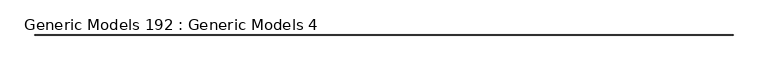
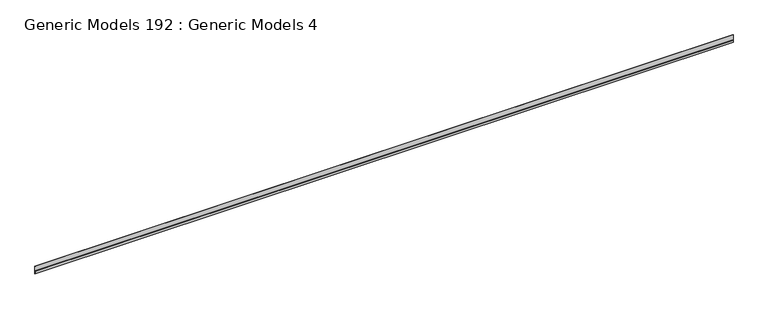
"""IFC4 building model written with IfcOpenShell, lengths in millimetres: proxy geometry, Generic Models 192 : Generic Models 4."""

import ifcopenshell
import ifcopenshell.guid

model = None  # the IFC model being written
_history = None  # IfcOwnerHistory: only IFC2X3 demands one
_inside = {}  # id of a spatial element -> (the spatial element, [elements in it])
_under = {}  # id of a project, library or spatial element -> (it, [spatial elements below it])
_declared = {}  # id of a project -> (the project, [libraries it declares])
_typed = {}  # id of a type object -> (the type object, [elements of that type])
_made_of = {}  # id of a material, layer set ... -> (it, [elements and type objects made of it])


def new_model(schema):
    """Start an empty IFC model of exactly this schema.

    Asked for "IFC4X3", IfcOpenShell would pick the latest addendum, in which some entities
    have other attributes; the version numbers below select the first issue.
    IFC2X3 requires an IfcOwnerHistory on every rooted entity: one is made here for all.
    """
    global model, _history
    if schema == "IFC4X3":
        model = ifcopenshell.file(schema_version=(4, 3, 0, 0))
    else:
        model = ifcopenshell.file(schema=schema)
    _inside.clear()
    _under.clear()
    _declared.clear()
    _typed.clear()
    _made_of.clear()
    _history = None
    if model.schema == "IFC2X3":
        org = make("IfcOrganization", Name="unknown")
        user = make(
            "IfcPersonAndOrganization",
            ThePerson=make("IfcPerson", FamilyName="unknown"),
            TheOrganization=org,
        )
        app = make(
            "IfcApplication",
            ApplicationDeveloper=org,
            Version="unknown",
            ApplicationFullName="unknown",
            ApplicationIdentifier="unknown",
        )
        _history = make(
            "IfcOwnerHistory",
            OwningUser=user,
            OwningApplication=app,
            ChangeAction="ADDED",
            CreationDate=0,
        )
    return model


def make(cls, **values):
    """One entity of the class cls with the attributes given. An attribute that is None is left unset."""
    return model.create_entity(
        cls, **{name: value for name, value in values.items() if value is not None}
    )


def rooted(cls, **values):
    """An entity with a GlobalId (a new one), such as an element, a storey or a relation."""
    return make(cls, GlobalId=ifcopenshell.guid.new(), OwnerHistory=_history, **values)


def si_unit(unit_type, name, prefix=None):
    """IfcSIUnit, for example si_unit("LENGTHUNIT", "METRE", prefix="MILLI")."""
    return make("IfcSIUnit", UnitType=unit_type, Prefix=prefix, Name=name)


def assignment(units):
    """IfcUnitAssignment: the units of a project."""
    return None if units is None else make("IfcUnitAssignment", Units=units)


def point(xyz):
    """IfcCartesianPoint."""
    return None if xyz is None else make("IfcCartesianPoint", Coordinates=xyz)


def direction(xyz):
    """IfcDirection."""
    return None if xyz is None else make("IfcDirection", DirectionRatios=xyz)


def frame(location, z_axis=None, x_axis=None):
    """IfcAxis2Placement3D, a coordinate frame: its origin and axes. An axis left out is left unset."""
    return make(
        "IfcAxis2Placement3D",
        Location=point(location),
        Axis=direction(z_axis),
        RefDirection=direction(x_axis),
    )


def origin():
    """The frame at (0, 0, 0) with its axes left unset."""
    return frame((0.0, 0.0, 0.0))


def place(relative_to, where):
    """IfcLocalPlacement: puts the frame where relative to a parent placement (None: the world)."""
    return make(
        "IfcLocalPlacement", PlacementRelTo=relative_to, RelativePlacement=where
    )


def context(
    kind, dimensions, precision=None, world=None, true_north=None, identifier=None
):
    """IfcGeometricRepresentationContext, for example the 3D "Model" context."""
    return make(
        "IfcGeometricRepresentationContext",
        ContextIdentifier=identifier,
        ContextType=kind,
        CoordinateSpaceDimension=dimensions,
        Precision=precision,
        WorldCoordinateSystem=world,
        TrueNorth=true_north,
    )


def project(units=None, contexts=None):
    """IfcProject with its units and contexts."""
    return rooted(
        "IfcProject",
        Name="project",
        RepresentationContexts=contexts,
        UnitsInContext=assignment(units),
    )


def spatial(cls, under=None, at=None, **own):
    """A site, building, storey or space (cls), placed at a placement, below another one or the project."""
    s = rooted(cls, ObjectPlacement=at, **own)
    if under is not None:
        _under.setdefault(under.id(), (under, []))[1].append(s)
    return s


def polyline(points):
    """IfcPolyline through the points."""
    return make("IfcPolyline", Points=[point(p) for p in points])


def outline(outer, holes=None, kind="AREA"):
    """IfcArbitraryClosedProfileDef: a profile drawn as a closed curve; with holes, ...WithVoids."""
    if holes is None:
        return make("IfcArbitraryClosedProfileDef", ProfileType=kind, OuterCurve=outer)
    return make(
        "IfcArbitraryProfileDefWithVoids",
        ProfileType=kind,
        OuterCurve=outer,
        InnerCurves=holes,
    )


def extrude(swept, where, along, depth):
    """IfcExtrudedAreaSolid: the profile swept, set in the frame where, extruded along a direction by depth."""
    return make(
        "IfcExtrudedAreaSolid",
        SweptArea=swept,
        Position=where,
        ExtrudedDirection=direction(along),
        Depth=depth,
    )


def shape(context_of_items, identifier, shape_type, items):
    """IfcShapeRepresentation: the items that make up one representation, for example the "Body"."""
    return make(
        "IfcShapeRepresentation",
        ContextOfItems=context_of_items,
        RepresentationIdentifier=identifier,
        RepresentationType=shape_type,
        Items=items,
    )


def source(mapping_origin, context_of_items, identifier, shape_type, items):
    """IfcRepresentationMap: a shape defined once, which mapped items show again and again."""
    return make(
        "IfcRepresentationMap",
        MappingOrigin=mapping_origin,
        MappedRepresentation=shape(context_of_items, identifier, shape_type, items),
    )


def transform(
    local_origin,
    x_axis=None,
    y_axis=None,
    z_axis=None,
    scale=None,
    scale2=None,
    scale3=None,
    uniform=True,
):
    """IfcCartesianTransformationOperator3D, or its non-uniform kind. x_axis, y_axis, z_axis: its Axis1, 2, 3."""
    if uniform:
        return make(
            "IfcCartesianTransformationOperator3D",
            Axis1=direction(x_axis),
            Axis2=direction(y_axis),
            LocalOrigin=point(local_origin),
            Scale=scale,
            Axis3=direction(z_axis),
        )
    return make(
        "IfcCartesianTransformationOperator3DnonUniform",
        Axis1=direction(x_axis),
        Axis2=direction(y_axis),
        LocalOrigin=point(local_origin),
        Scale=scale,
        Axis3=direction(z_axis),
        Scale2=scale2,
        Scale3=scale3,
    )


def mapped(mapping_source, mapping_target):
    """IfcMappedItem: shows the shape of a source again, moved by a transform."""
    return make(
        "IfcMappedItem", MappingSource=mapping_source, MappingTarget=mapping_target
    )


def made_of(thing, what):
    """Note that an element or type object is made of a material, layer set ...; save() writes the relation."""
    if what is not None:
        _made_of.setdefault(what.id(), (what, []))[1].append(thing)
    return thing


def element(
    cls,
    number,
    at=None,
    inside=None,
    cuts=None,
    type_object=None,
    material=None,
    context=None,
    identifier="Body",
    shape_type=None,
    held_by="IfcProductDefinitionShape",
    body=None,
    shapes=None,
    **own,
):
    """One element of the class cls, such as IfcWall. Its Tag is "e" and its number.

    at: its placement. inside: the storey or other place that contains it. cuts: it is an
    opening in that element (IfcRelVoidsElement). A single representation is given by context,
    identifier, shape_type and body (its items); several are given by shapes. held_by: the class
    of the entity that holds the representations. save() writes the other relations.
    """
    e = rooted(cls, Tag="e%d" % number, ObjectPlacement=at, **own)
    if body is not None:
        shapes = [shape(context, identifier, shape_type, body)]
    if shapes is not None:
        e.Representation = make(held_by, Representations=shapes)
    if inside is not None:
        _inside.setdefault(inside.id(), (inside, []))[1].append(e)
    if cuts is not None:
        rooted(
            "IfcRelVoidsElement", RelatingBuildingElement=cuts, RelatedOpeningElement=e
        )
    if type_object is not None:
        _typed.setdefault(type_object.id(), (type_object, []))[1].append(e)
    return made_of(e, material)


def aggregate(whole, parts):
    """IfcRelAggregates: a whole, such as a stair, and the parts it consists of."""
    return rooted("IfcRelAggregates", RelatingObject=whole, RelatedObjects=parts)


def save(model, path):
    """Write the relations noted so far, then the file.

    IfcRelAggregates (storeys below a building ...), IfcRelContainedInSpatialStructure (elements
    in a storey), IfcRelDefinesByType, IfcRelAssociatesMaterial and IfcRelDeclares: one each for
    every whole, place, type object, material and project.
    """
    for whole, parts in _under.values():
        aggregate(whole, parts)
    for where, things in _inside.values():
        rooted(
            "IfcRelContainedInSpatialStructure",
            RelatedElements=things,
            RelatingStructure=where,
        )
    for kind, things in _typed.values():
        rooted("IfcRelDefinesByType", RelatedObjects=things, RelatingType=kind)
    for what, things in _made_of.values():
        rooted("IfcRelAssociatesMaterial", RelatedObjects=things, RelatingMaterial=what)
    for by, libraries in _declared.values():
        rooted("IfcRelDeclares", RelatingContext=by, RelatedDefinitions=libraries)
    model.write(path)


def generic_models_192_generic_models_4_7e6c567b(model_context):
    return source(origin(), model_context, "Body", "SweptSolid", [
        extrude(outline(polyline([(-5470.6218745, 127034.2936598), (-5472.9098421, 127024.3833833), (-5472.9098421, 126982.7011354), (-5473.7035921, 126982.7011354), (-5473.7035921, 127024.4738197), (-5471.4156245, 127034.3840962), (-5471.4156245, 127122.7316067), (-5470.6218745, 127122.7316067), (-5470.6218745, 127034.2936598)])), frame((-10234.5171316, 0.0, 0.0), z_axis=(1.0, 0.0, 0.0), x_axis=(0.0, 1.0, 0.0)), (0.0, 0.0, 1.0), 12431.443502),
    ])


if __name__ == "__main__":
    model = new_model("IFC4")
    model_context = context("Model", 3, world=origin())
    ifc_project = project(units=[si_unit("LENGTHUNIT", "METRE", prefix="MILLI")], contexts=[model_context])
    site = spatial("IfcSite", under=ifc_project)
    building = spatial("IfcBuilding", under=site)
    placement = place(None, origin())
    generic_models_192_generic_models_4_shape = generic_models_192_generic_models_4_7e6c567b(model_context)
    element("IfcBuildingElementProxy", 1, Name="Generic Models 192 : Generic Models 4", ObjectType="Generic Models 192 : Generic Models 4", at=placement, inside=building, context=model_context, shape_type="MappedRepresentation", body=[
        mapped(generic_models_192_generic_models_4_shape, transform((0.0, 0.0, 0.0), x_axis=(1.0, 0.0, 0.0), y_axis=(0.0, 1.0, 0.0), z_axis=(0.0, 0.0, 1.0))),
    ])
    save(model, "model.ifc")

# Revit data of these elements
# Element 1 (IfcBuildingElementProxy, "Generic Models 192 : Generic Models 4")
#   Materials on its faces: "_(2) LAYERS NO. 30 ASTM D226 ASPHALT SATURATED ORGANIC FELT"
# Materials
#   "_(2) LAYERS NO. 30 ASTM D226 ASPHALT SATURATED ORGANIC FELT": class "Generic", colour RGB 67 154 161, transparency 0, Cost = 0
